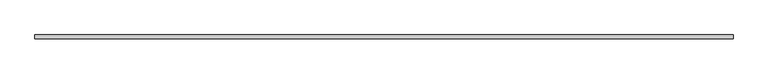
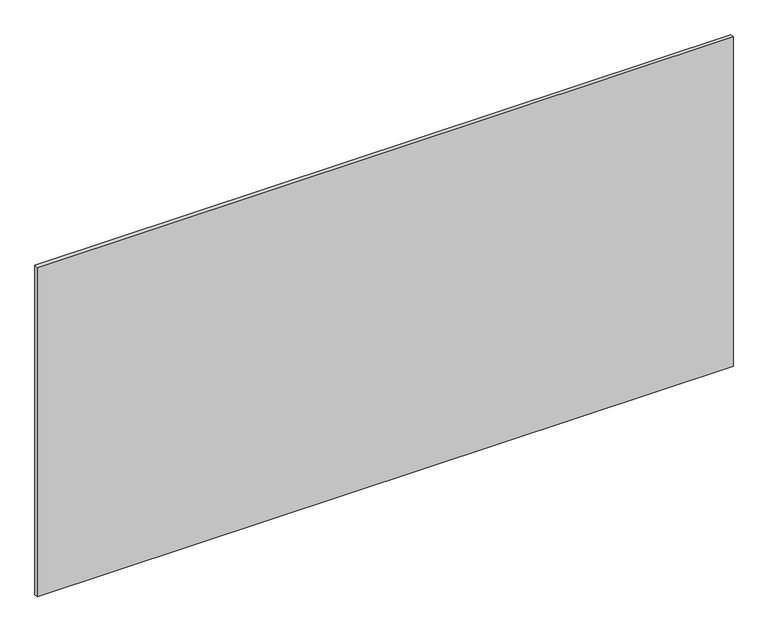
"""IFC4 building model written with IfcOpenShell, lengths in millimetres: proxy geometry, Inner panel:Inner panel:1:Inner panel:1 : Inner panel:Inner panel:300324:300043:Inner panel:1:Inner panel:1 : Inner panel:Inner panel:300324:300043 : Inner panel:Inner panel:1:Inner panel:1 : Inner panel:Inner panel:300324:300043:10 : Inner panel:Inner panel:1:Inner panel:1 : Inner panel:Inner panel:300324:300043:Inner panel:1:Inner panel:1 : Inner panel:Inner panel:300324:300043 : Inner panel:Inner panel:1:Inner panel:1 : Inner panel:Inner panel:300324:300043:300031."""

from ifc_helpers import new_model, si_unit, frame, origin, place, context, project, spatial, polyline, outline, extrude, source, transform, mapped, element, save


def generic_models_9c2322f1(model_context):
    return source(origin(), model_context, "Body", "SweptSolid", [
        extrude(outline(polyline([(570452.6367239, -579000.6913841), (572891.0367239, -579000.6913841), (572891.0367239, -579013.3913841), (570452.6367239, -579013.3913841), (570452.6367239, -579000.6913841)])), frame((0.0, 0.0, 4946.65), z_axis=(0.0, 0.0, 1.0), x_axis=(1.0, 0.0, 0.0)), (0.0, 0.0, 1.0), 1219.2),
    ])


if __name__ == "__main__":
    model = new_model("IFC4")
    model_context = context("Model", 3, world=origin())
    ifc_project = project(units=[si_unit("LENGTHUNIT", "METRE", prefix="MILLI")], contexts=[model_context])
    site = spatial("IfcSite", under=ifc_project)
    building = spatial("IfcBuilding", under=site)
    placement = place(None, origin())
    generic_models_shape = generic_models_9c2322f1(model_context)
    element("IfcBuildingElementProxy", 1, Name="Inner panel:Inner panel:1:Inner panel:1 : Inner panel:Inner panel:300324:300043:Inner panel:1:Inner panel:1 : Inner panel:Inner panel:300324:300043 : Inner panel:Inner panel:1:Inner panel:1 : Inner panel:Inner panel:300324:300043:10 : Inner panel:Inner panel:1:Inner panel:1 : Inner panel:Inner panel:300324:300043:Inner panel:1:Inner panel:1 : Inner panel:Inner panel:300324:300043 : Inner panel:Inner panel:1:Inner panel:1 : Inner panel:Inner panel:300324:300043:300031", ObjectType="Inner panel:Inner panel:1:Inner panel:1 : Inner panel:Inner panel:300324:300043:Inner panel:1:Inner panel:1 : Inner panel:Inner panel:300324:300043 : Inner panel:Inner panel:1:Inner panel:1 : Inner panel:Inner panel:300324:300043:10 : Inner panel:Inner panel:1:Inner panel:1 : Inner panel:Inner panel:300324:300043:Inner panel:1:Inner panel:1 : Inner panel:Inner panel:300324:300043 : Inner panel:Inner panel:1:Inner panel:1 : Inner panel:Inner panel:300324:300043:300031", at=placement, inside=building, context=model_context, shape_type="MappedRepresentation", body=[
        mapped(generic_models_shape, transform((0.0, 0.0, 0.0), x_axis=(1.0, 0.0, 0.0), y_axis=(0.0, 1.0, 0.0), z_axis=(0.0, 0.0, 1.0))),
    ])
    save(model, "model.ifc")

# Revit data of these elements
# Type "Inner panel:Inner panel:1:Inner panel:1 : Inner panel:Inner panel:300324:300043:Inner panel:1:Inner panel:1 : Inner panel:Inner panel:300324:300043 : Inner panel:Inner panel:1:Inner panel:1 : Inner panel:Inner panel:300324:300043:10 : Inner panel:Inner panel:1:Inner panel:1 : Inner panel:Inner panel:300324:300043:Inner panel:1:Inner panel:1 : Inner panel:Inner panel:300324:300043 : Inner panel:Inner panel:1:Inner panel:1 : Inner panel:Inner panel:300324:300043:300031"
#   NameOverride = "Inner panel:Inner panel:1:Inner panel:1 : Inner panel:Inner panel:300324:300043:Inner panel:1:Inner panel:1 : Inner panel:Inner panel:300324:300043 : Inner panel:Inner panel:1:Inner panel:1 : Inner panel:Inner panel:300324:300043:300031"
#   ObjectTypeOverride = "Inner panel:1:Inner panel:1 : Inner panel:Inner panel:300324:300043 : Inner panel:Inner panel:1:Inner panel:1 : Inner panel:Inner panel:300324:300043"
#   Reference = "Inner panel"
#   Tag = "300031"
# Element 1 (IfcBuildingElementProxy, "Inner panel:Inner panel:1:Inner panel:1 : Inner panel:Inner panel:300324:300043:Inner panel:1:Inner panel:1 : Inner panel:Inner panel:300324:300043 : Inner panel:Inner panel:1:Inner panel:1 : Inner panel:Inner panel:300324:300043:10 : Inner panel:Inner panel:1:Inner panel:1 : Inner panel:Inner panel:300324:300043:Inner panel:1:Inner panel:1 : Inner panel:Inner panel:300324:300043 : Inner panel:Inner panel:1:Inner panel:1 : Inner panel:Inner panel:300324:300043:300031")
#   Materials on its faces: "1/2\" EXTERIOR GRADE FIRE RETARDANT CDX PLYWOOD"
# Materials
#   "1/2\" EXTERIOR GRADE FIRE RETARDANT CDX PLYWOOD": class "Unassigned", colour RGB 196 177 123, transparency 0, Cost = 0
